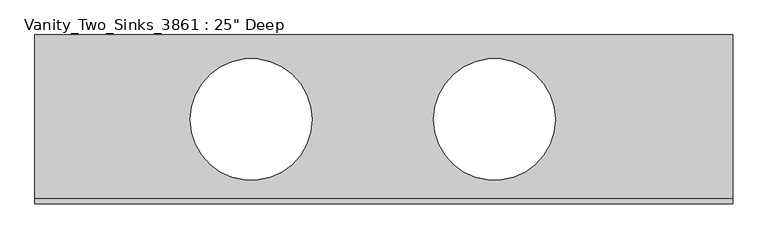
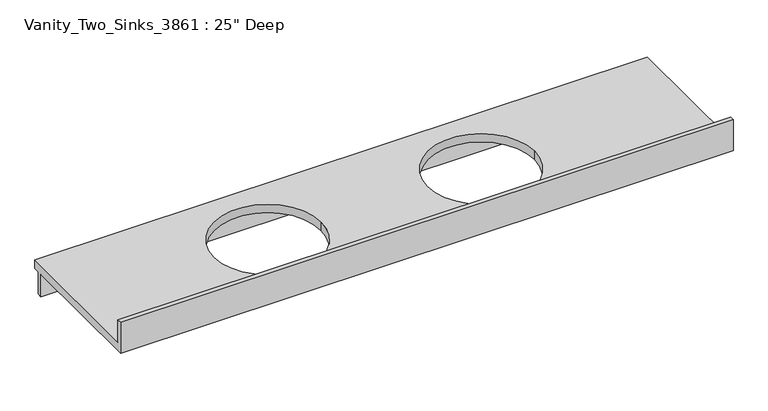
"""IFC4 building model written with IfcOpenShell, lengths in millimetres: furniture geometry."""

from ifc_helpers import new_model, si_unit, frame, origin, place, context, project, spatial, polyline, circle_curve, source, transform, mapped, element, save
from ifc_brep_helpers import plane_surface, revolved_surface, advanced_brep


def furniture_a1511c22(model_context):
    return source(origin(), model_context, "Body", "AdvancedBrep", [
        advanced_brep(
        [(-1327.4622951, 635.0, 863.6), (-1327.4622951, 19.05, 863.6), (1295.0877049, 19.05, 863.6), (1295.0877049, 635.0, 863.6), (628.3736357, 317.5, 863.6), (171.1736357, 317.5, 863.6), (-286.0263643, 317.5, 863.6), (-743.2263643, 317.5, 863.6), (1295.0877049, 635.0, 825.5), (1295.0877049, 609.6, 825.5), (-1327.4622951, 609.6, 825.5), (-1327.4622951, 635.0, 825.5), (-1327.4622951, 0.0, 825.5), (-1327.4622951, 590.55, 825.5), (1295.0877049, 590.55, 825.5), (1295.0877049, 0.0, 825.5), (171.1736357, 317.5, 825.5), (628.3736357, 317.5, 825.5), (-743.2263643, 317.5, 825.5), (-286.0263643, 317.5, 825.5), (1295.0877049, 0.0, 965.2), (-1327.4622951, 0.0, 965.2), (-1327.4622951, 609.6, 723.9), (-1327.4622951, 590.55, 723.9), (-1327.4622951, 19.05, 965.2), (1295.0877049, 19.05, 965.2), (1295.0877049, 590.55, 723.9), (1295.0877049, 609.6, 723.9)],
        [
            (0, 1),
            (1, 2),
            (2, 3),
            (3, 0),
            (4, 5, circle_curve(frame((399.7736357, 317.5, 863.6), z_axis=(0.0, 0.0, -1.0), x_axis=(1.0, 0.0, 0.0)), 228.6)),
            (5, 4, circle_curve(frame((399.7736357, 317.5, 863.6), z_axis=(0.0, 0.0, -1.0), x_axis=(1.0, 0.0, 0.0)), 228.6)),
            (6, 7, circle_curve(frame((-514.6263643, 317.5, 863.6), z_axis=(0.0, 0.0, -1.0), x_axis=(1.0, 0.0, 0.0)), 228.6)),
            (7, 6, circle_curve(frame((-514.6263643, 317.5, 863.6), z_axis=(0.0, 0.0, -1.0), x_axis=(1.0, 0.0, 0.0)), 228.6)),
            (8, 9),
            (9, 10),
            (10, 11),
            (11, 8),
            (12, 13),
            (13, 14),
            (14, 15),
            (15, 12),
            (16, 17, circle_curve(frame((399.7736357, 317.5, 825.5), z_axis=(0.0, 0.0, 1.0), x_axis=(1.0, 0.0, 0.0)), 228.6)),
            (17, 16, circle_curve(frame((399.7736357, 317.5, 825.5), z_axis=(0.0, 0.0, 1.0), x_axis=(1.0, 0.0, 0.0)), 228.6)),
            (18, 19, circle_curve(frame((-514.6263643, 317.5, 825.5), z_axis=(0.0, 0.0, 1.0), x_axis=(1.0, 0.0, 0.0)), 228.6)),
            (19, 18, circle_curve(frame((-514.6263643, 317.5, 825.5), z_axis=(0.0, 0.0, 1.0), x_axis=(1.0, 0.0, 0.0)), 228.6)),
            (15, 20),
            (20, 21),
            (21, 12),
            (10, 22),
            (22, 23),
            (23, 13),
            (21, 24),
            (24, 1),
            (0, 11),
            (3, 8),
            (2, 25),
            (25, 20),
            (14, 26),
            (26, 27),
            (27, 9),
            (5, 16),
            (17, 4),
            (25, 24),
            (7, 18),
            (19, 6),
            (26, 23),
            (22, 27),
        ],
        [
            plane_surface(frame((-1327.4622951, 0.0, 863.6), z_axis=(0.0, 0.0, 1.0), x_axis=(-1.0, 0.0, 0.0))),
            plane_surface(frame((-1327.4622951, 0.0, 825.5), z_axis=(0.0, 0.0, -1.0), x_axis=(1.0, 0.0, 0.0))),
            plane_surface(frame((1295.0877049, 0.0, 863.6), z_axis=(0.0, -1.0, 0.0), x_axis=(0.0, 0.0, -1.0))),
            plane_surface(frame((-1327.4622951, 0.0, 863.6), z_axis=(-1.0, 0.0, 0.0), x_axis=(0.0, 0.0, -1.0))),
            plane_surface(frame((-1327.4622951, 635.0, 863.6), z_axis=(0.0, 1.0, 0.0), x_axis=(0.0, 0.0, -1.0))),
            plane_surface(frame((1295.0877049, 635.0, 863.6), z_axis=(1.0, 0.0, 0.0), x_axis=(0.0, 0.0, -1.0))),
            revolved_surface(polyline([(628.3736357, 317.5, 863.6), (628.3736357, 317.5, 825.5)]), (399.7736357, 317.5, 825.5), (0.0, 0.0, 1.0)),
            plane_surface(frame((-1327.4622951, 0.0, 965.2), z_axis=(0.0, 0.0, 1.0), x_axis=(0.0, 1.0, 0.0))),
            plane_surface(frame((-1327.4622951, 19.05, 965.2), z_axis=(0.0, 1.0, 0.0), x_axis=(0.0, 0.0, -1.0))),
            revolved_surface(polyline([(-286.02636429999995, 317.5, 863.6), (-286.02636429999995, 317.5, 825.5)]), (-514.6263643, 317.5, 825.5), (0.0, 0.0, 1.0)),
            plane_surface(frame((-1327.4622951, 590.55, 723.9), z_axis=(0.0, 0.0, -1.0), x_axis=(1.0, 0.0, 0.0))),
            plane_surface(frame((1295.0877049, 590.55, 825.5), z_axis=(0.0, -1.0, 0.0), x_axis=(0.0, 0.0, -1.0))),
            plane_surface(frame((-1327.4622951, 609.6, 825.5), z_axis=(0.0, 1.0, 0.0), x_axis=(0.0, 0.0, -1.0))),
        ],
        [
            (0, [[1, 2, 3, 4], [5, 6], [7, 8]]),
            (1, [[9, 10, 11, 12]]),
            (1, [[13, 14, 15, 16], [17, 18], [19, 20]]),
            (2, [[21, 22, 23, -16]]),
            (3, [[-11, 24, 25, 26, -13, -23, 27, 28, -1, 29]]),
            (4, [[30, -12, -29, -4]]),
            (5, [[-3, 31, 32, -21, -15, 33, 34, 35, -9, -30]]),
            (6, [[-6, 36, -18, 37]]),
            (6, [[-17, -36, -5, -37]]),
            (7, [[-22, -32, 38, -27]]),
            (8, [[-31, -2, -28, -38]]),
            (9, [[-8, 39, -20, 40]]),
            (9, [[-19, -39, -7, -40]]),
            (10, [[41, -25, 42, -34]]),
            (11, [[-33, -14, -26, -41]]),
            (12, [[-24, -10, -35, -42]]),
        ],
    ),
    ])


if __name__ == "__main__":
    model = new_model("IFC4")
    model_context = context("Model", 3, world=origin())
    ifc_project = project(units=[si_unit("LENGTHUNIT", "METRE", prefix="MILLI")], contexts=[model_context])
    site = spatial("IfcSite", under=ifc_project)
    building = spatial("IfcBuilding", under=site)
    placement = place(None, origin())
    furniture_shape = furniture_a1511c22(model_context)
    element("IfcFurniture", 1, ObjectType="Vanity_Two_Sinks_3861 : 25\" Deep", at=placement, inside=building, context=model_context, shape_type="MappedRepresentation", body=[
        mapped(furniture_shape, transform((0.0, 0.0, 0.0), x_axis=(1.0, 0.0, 0.0), y_axis=(0.0, 1.0, 0.0), z_axis=(0.0, 0.0, 1.0))),
    ])
    save(model, "model.ifc")

# Revit data of these elements
# Type "Vanity_Two_Sinks_3861 : 25\" Deep"
#   Assembly Code = "C1030400"
#   Sink Location Right [instance default] = 1' - 6"
#   Counter Thickness = 0' - 1 1/2"
#   Depth = 2' - 1"
#   Height = 2' - 10"
#   Length [instance default] = 6' - 0"
#   Sink Location Left [instance default] = 1' - 6"
#   Sink to Back Wall = 0' - 4"
#   Sink Opening Width [instance default] = 1' - 5"
#   Counter Top = Casework - Vanity Top
#   Width = 0
# Element 1 (IfcFurniture, "Vanity_Two_Sinks_3861 : 25\" Deep")
#   Sink Location Right = 2' - 11.24859"
#   Length = 8' - 7 1/4"
#   Sink Location Left = 2' - 8.00141"
#   Materials on its faces: "Casework - Vanity Top"
# Materials
#   "Casework - Vanity Top": class "Unassigned", colour RGB 210 200 171, transparency 0, Comments = "Rendering appearance not upgraded "
